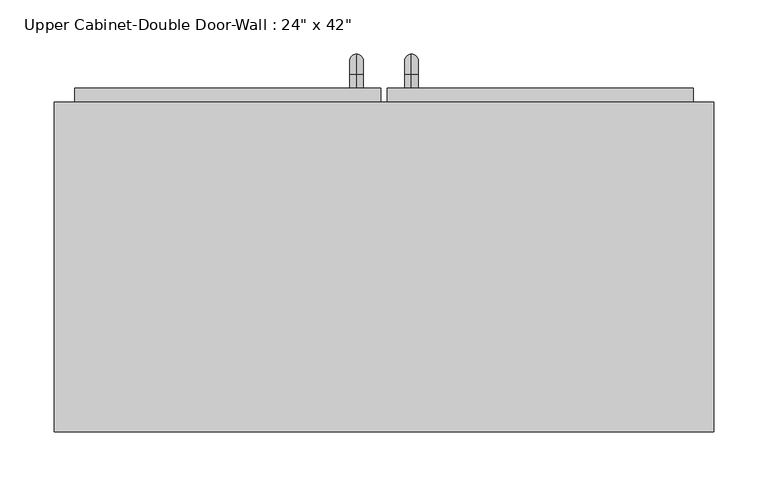
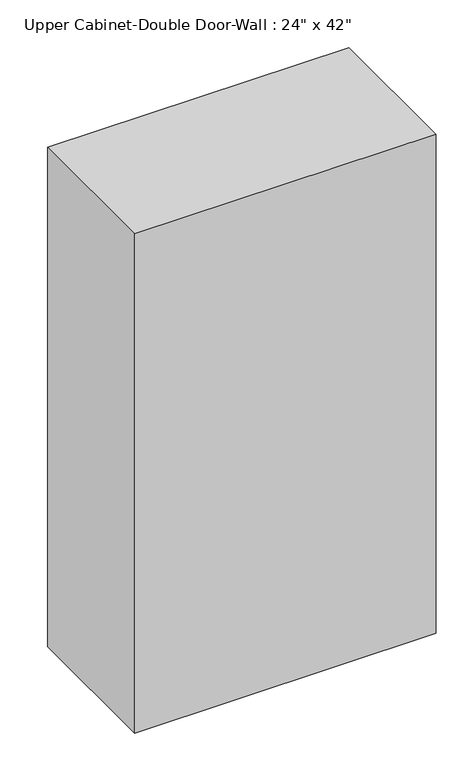
"""IFC4 building model written with IfcOpenShell, lengths in millimetres: furniture geometry."""

from ifc_helpers import new_model, si_unit, point, frame, origin, place, context, project, spatial, polyline, circle_curve, ellipse_curve, trimmed, outline, extrude, faceted_brep, source, transform, mapped, element, save
from ifc_brep_helpers import plane_surface, cylinder_surface, revolved_surface, advanced_brep


def furniture_7ad92d76(model_context):
    return source(origin(), model_context, "Body", "SolidModel", [
        faceted_brep([(-275.0288372, 61.9125, 2438.4), (-275.0288372, 61.9125, 1371.6), (334.5711628, 61.9125, 1371.6), (334.5711628, 61.9125, 2438.4), (-275.0288372, 366.7125, 2438.4), (334.5711628, 366.7125, 2438.4), (334.5711628, 366.7125, 1371.6), (-275.0288372, 366.7125, 1371.6), (-255.9788372, 366.7125, 2419.35), (-255.9788372, 366.7125, 1390.65), (315.5211628, 366.7125, 1390.65), (315.5211628, 366.7125, 2419.35), (315.5211628, 80.9625, 2419.35), (-255.9788372, 80.9625, 2419.35), (315.5211628, 80.9625, 1390.65), (-255.9788372, 80.9625, 1390.65)], [[[0, 1, 2, 3]], [[4, 5, 6, 7], [8, 9, 10, 11]], [[1, 0, 4, 7]], [[2, 1, 7, 6]], [[3, 2, 6, 5]], [[0, 3, 5, 4]], [[8, 11, 12, 13]], [[11, 10, 14, 12]], [[10, 9, 15, 14]], [[9, 8, 13, 15]], [[13, 12, 14, 15]]]),
        advanced_brep(
        [(55.1711628, 379.4125, 1517.65), (55.1711628, 379.4125, 1530.35), (55.1711628, 392.1125, 1517.65), (55.1711628, 392.1125, 1530.35), (55.1711628, 411.1625, 1511.3), (55.1711628, 398.4625, 1511.3), (55.1711628, 398.4625, 1435.1), (55.1711628, 411.1625, 1435.1), (55.1711628, 392.1125, 1416.05), (55.1711628, 392.1125, 1428.75), (55.1711628, 379.4125, 1428.75), (55.1711628, 379.4125, 1416.05)],
        [
            (0, 1, circle_curve(frame((55.1711628, 379.4125, 1524.0), z_axis=(0.0, -1.0, 0.0), x_axis=(0.0, 0.0, -1.0)), 6.35)),
            (1, 0, circle_curve(frame((55.1711628, 379.4125, 1524.0), z_axis=(0.0, -1.0, 0.0), x_axis=(0.0, 0.0, -1.0)), 6.35)),
            (0, 2),
            (2, 3, circle_curve(frame((55.1711628, 392.1125, 1524.0), z_axis=(0.0, -1.0, 0.0), x_axis=(0.0, 0.0, -1.0)), 6.35)),
            (3, 1),
            (3, 2, circle_curve(frame((55.1711628, 392.1125, 1524.0), z_axis=(0.0, -1.0, 0.0), x_axis=(0.0, 0.0, -1.0)), 6.35)),
            (4, 3, circle_curve(frame((55.1711628, 392.1125, 1511.3), z_axis=(1.0, 0.0, 0.0), x_axis=(0.0, 0.0, 1.0)), 19.05)),
            (2, 5, circle_curve(frame((55.1711628, 392.1125, 1511.3), z_axis=(-1.0, 0.0, 0.0), x_axis=(0.0, 0.0, 1.0)), 6.35)),
            (5, 4, circle_curve(frame((55.1711628, 404.8125, 1511.3), z_axis=(0.0, 0.0, 1.0), x_axis=(0.0, -1.0, 0.0)), 6.35)),
            (4, 5, circle_curve(frame((55.1711628, 404.8125, 1511.3), z_axis=(0.0, 0.0, 1.0), x_axis=(0.0, -1.0, 0.0)), 6.35)),
            (5, 6),
            (6, 7, circle_curve(frame((55.1711628, 404.8125, 1435.1), z_axis=(0.0, 0.0, 1.0), x_axis=(0.0, -1.0, 0.0)), 6.35)),
            (7, 4),
            (7, 6, circle_curve(frame((55.1711628, 404.8125, 1435.1), z_axis=(0.0, 0.0, 1.0), x_axis=(0.0, -1.0, 0.0)), 6.35)),
            (8, 7, circle_curve(frame((55.1711628, 392.1125, 1435.1), z_axis=(1.0, 0.0, 0.0), x_axis=(0.0, 1.0, 0.0)), 19.05)),
            (6, 9, circle_curve(frame((55.1711628, 392.1125, 1435.1), z_axis=(-1.0, 0.0, 0.0), x_axis=(0.0, 1.0, 0.0)), 6.35)),
            (9, 8, circle_curve(frame((55.1711628, 392.1125, 1422.4), z_axis=(0.0, 1.0, 0.0), x_axis=(0.0, 0.0, 1.0)), 6.35)),
            (8, 9, circle_curve(frame((55.1711628, 392.1125, 1422.4), z_axis=(0.0, 1.0, 0.0), x_axis=(0.0, 0.0, 1.0)), 6.35)),
            (10, 11, circle_curve(frame((55.1711628, 379.4125, 1422.4), z_axis=(0.0, -1.0, 0.0), x_axis=(0.0, 0.0, 1.0)), 6.35)),
            (11, 10, circle_curve(frame((55.1711628, 379.4125, 1422.4), z_axis=(0.0, -1.0, 0.0), x_axis=(0.0, 0.0, 1.0)), 6.35)),
            (9, 10),
            (11, 8),
        ],
        [
            plane_surface(frame((48.8211628, 379.4125, 1524.0), z_axis=(0.0, -1.0, 0.0), x_axis=(0.0, 0.0, 1.0))),
            cylinder_surface(frame((55.1711628, 379.4125, 1524.0), z_axis=(0.0, -1.0, 0.0), x_axis=(0.0, 0.0, -1.0)), 6.35),
            revolved_surface(trimmed(ellipse_curve(frame((55.1711628, 392.1125, 1524.0), z_axis=(0.0, -1.0, 0.0), x_axis=(0.0, 0.0, -1.0)), 6.35, 6.35), [point((55.1711628, 392.1125, 1517.65))], [point((55.1711628, 392.1125, 1530.35))], True, "CARTESIAN"), (55.1711628, 392.1125, 1511.3), (-1.0, 0.0, 0.0)),
            revolved_surface(trimmed(ellipse_curve(frame((55.1711628, 392.1125, 1524.0), z_axis=(0.0, -1.0, 0.0), x_axis=(0.0, 0.0, -1.0)), 6.35, 6.35), [point((55.1711628, 392.1125, 1530.35))], [point((55.1711628, 392.1125, 1517.65))], True, "CARTESIAN"), (55.1711628, 392.1125, 1511.3), (-1.0, 0.0, 0.0)),
            cylinder_surface(frame((55.1711628, 404.8125, 1511.3), z_axis=(0.0, 0.0, 1.0), x_axis=(0.0, -1.0, 0.0)), 6.35),
            revolved_surface(trimmed(ellipse_curve(frame((55.1711628, 404.8125, 1435.1), z_axis=(0.0, 0.0, 1.0), x_axis=(0.0, -1.0, 0.0)), 6.35, 6.35), [point((55.1711628, 398.4625, 1435.1))], [point((55.1711628, 411.1625, 1435.1))], True, "CARTESIAN"), (55.1711628, 392.1125, 1435.1), (-1.0, 0.0, 0.0)),
            revolved_surface(trimmed(ellipse_curve(frame((55.1711628, 404.8125, 1435.1), z_axis=(0.0, 0.0, 1.0), x_axis=(0.0, -1.0, 0.0)), 6.35, 6.35), [point((55.1711628, 411.1625, 1435.1))], [point((55.1711628, 398.4625, 1435.1))], True, "CARTESIAN"), (55.1711628, 392.1125, 1435.1), (-1.0, 0.0, 0.0)),
            plane_surface(frame((48.8211628, 379.4125, 1422.4), z_axis=(0.0, -1.0, 0.0), x_axis=(0.0, 0.0, -1.0))),
            cylinder_surface(frame((55.1711628, 392.1125, 1422.4), z_axis=(0.0, 1.0, 0.0), x_axis=(0.0, 0.0, 1.0)), 6.35),
        ],
        [
            (0, [[1, 2]]),
            (1, [[-1, 3, 4, 5]]),
            (1, [[-2, -5, 6, -3]]),
            (2, [[7, -4, 8, 9]]),
            (3, [[-8, -6, -7, 10]]),
            (4, [[-9, 11, 12, 13]]),
            (4, [[-10, -13, 14, -11]]),
            (5, [[15, -12, 16, 17]]),
            (6, [[-16, -14, -15, 18]]),
            (7, [[19, 20]]),
            (8, [[-17, 21, -20, 22]]),
            (8, [[-18, -22, -19, -21]]),
        ],
    ),
        advanced_brep(
        [(4.3711628, 379.4125, 1517.65), (4.3711628, 379.4125, 1530.35), (4.3711628, 392.1125, 1517.65), (4.3711628, 392.1125, 1530.35), (4.3711628, 411.1625, 1511.3), (4.3711628, 398.4625, 1511.3), (4.3711628, 398.4625, 1435.1), (4.3711628, 411.1625, 1435.1), (4.3711628, 392.1125, 1416.05), (4.3711628, 392.1125, 1428.75), (4.3711628, 379.4125, 1428.75), (4.3711628, 379.4125, 1416.05)],
        [
            (0, 1, circle_curve(frame((4.3711628, 379.4125, 1524.0), z_axis=(0.0, -1.0, 0.0), x_axis=(0.0, 0.0, 1.0)), 6.35)),
            (1, 0, circle_curve(frame((4.3711628, 379.4125, 1524.0), z_axis=(0.0, -1.0, 0.0), x_axis=(0.0, 0.0, 1.0)), 6.35)),
            (0, 2),
            (2, 3, circle_curve(frame((4.3711628, 392.1125, 1524.0), z_axis=(0.0, -1.0, 0.0), x_axis=(0.0, 0.0, 1.0)), 6.35)),
            (3, 1),
            (3, 2, circle_curve(frame((4.3711628, 392.1125, 1524.0), z_axis=(0.0, -1.0, 0.0), x_axis=(0.0, 0.0, 1.0)), 6.35)),
            (4, 3, circle_curve(frame((4.3711628, 392.1125, 1511.3), z_axis=(1.0, 0.0, 0.0), x_axis=(0.0, 0.0, 1.0)), 19.05)),
            (2, 5, circle_curve(frame((4.3711628, 392.1125, 1511.3), z_axis=(-1.0, 0.0, 0.0), x_axis=(0.0, 0.0, 1.0)), 6.35)),
            (5, 4, circle_curve(frame((4.3711628, 404.8125, 1511.3), z_axis=(0.0, 0.0, 1.0), x_axis=(0.0, 1.0, 0.0)), 6.35)),
            (4, 5, circle_curve(frame((4.3711628, 404.8125, 1511.3), z_axis=(0.0, 0.0, 1.0), x_axis=(0.0, 1.0, 0.0)), 6.35)),
            (5, 6),
            (6, 7, circle_curve(frame((4.3711628, 404.8125, 1435.1), z_axis=(0.0, 0.0, 1.0), x_axis=(0.0, 1.0, 0.0)), 6.35)),
            (7, 4),
            (7, 6, circle_curve(frame((4.3711628, 404.8125, 1435.1), z_axis=(0.0, 0.0, 1.0), x_axis=(0.0, 1.0, 0.0)), 6.35)),
            (8, 7, circle_curve(frame((4.3711628, 392.1125, 1435.1), z_axis=(1.0, 0.0, 0.0), x_axis=(0.0, 1.0, 0.0)), 19.05)),
            (6, 9, circle_curve(frame((4.3711628, 392.1125, 1435.1), z_axis=(-1.0, 0.0, 0.0), x_axis=(0.0, 1.0, 0.0)), 6.35)),
            (9, 8, circle_curve(frame((4.3711628, 392.1125, 1422.4), z_axis=(0.0, 1.0, 0.0), x_axis=(0.0, 0.0, -1.0)), 6.35)),
            (8, 9, circle_curve(frame((4.3711628, 392.1125, 1422.4), z_axis=(0.0, 1.0, 0.0), x_axis=(0.0, 0.0, -1.0)), 6.35)),
            (10, 11, circle_curve(frame((4.3711628, 379.4125, 1422.4), z_axis=(0.0, -1.0, 0.0), x_axis=(0.0, 0.0, -1.0)), 6.35)),
            (11, 10, circle_curve(frame((4.3711628, 379.4125, 1422.4), z_axis=(0.0, -1.0, 0.0), x_axis=(0.0, 0.0, -1.0)), 6.35)),
            (9, 10),
            (11, 8),
        ],
        [
            plane_surface(frame((-1.9788372, 379.4125, 1524.0), z_axis=(0.0, -1.0, 0.0), x_axis=(0.0, 0.0, 1.0))),
            cylinder_surface(frame((4.3711628, 379.4125, 1524.0), z_axis=(0.0, -1.0, 0.0), x_axis=(0.0, 0.0, 1.0)), 6.35),
            revolved_surface(trimmed(ellipse_curve(frame((4.3711628, 392.1125, 1524.0), z_axis=(0.0, -1.0, 0.0), x_axis=(0.0, 0.0, 1.0)), 6.35, 6.35), [point((4.3711628, 392.1125, 1517.65))], [point((4.3711628, 392.1125, 1530.35))], True, "CARTESIAN"), (4.3711628, 392.1125, 1511.3), (-1.0, 0.0, 0.0)),
            revolved_surface(trimmed(ellipse_curve(frame((4.3711628, 392.1125, 1524.0), z_axis=(0.0, -1.0, 0.0), x_axis=(0.0, 0.0, 1.0)), 6.35, 6.35), [point((4.3711628, 392.1125, 1530.35))], [point((4.3711628, 392.1125, 1517.65))], True, "CARTESIAN"), (4.3711628, 392.1125, 1511.3), (-1.0, 0.0, 0.0)),
            cylinder_surface(frame((4.3711628, 404.8125, 1511.3), z_axis=(0.0, 0.0, 1.0), x_axis=(0.0, 1.0, 0.0)), 6.35),
            revolved_surface(trimmed(ellipse_curve(frame((4.3711628, 404.8125, 1435.1), z_axis=(0.0, 0.0, 1.0), x_axis=(0.0, 1.0, 0.0)), 6.35, 6.35), [point((4.3711628, 398.4625, 1435.1))], [point((4.3711628, 411.1625, 1435.1))], True, "CARTESIAN"), (4.3711628, 392.1125, 1435.1), (-1.0, 0.0, 0.0)),
            revolved_surface(trimmed(ellipse_curve(frame((4.3711628, 404.8125, 1435.1), z_axis=(0.0, 0.0, 1.0), x_axis=(0.0, 1.0, 0.0)), 6.35, 6.35), [point((4.3711628, 411.1625, 1435.1))], [point((4.3711628, 398.4625, 1435.1))], True, "CARTESIAN"), (4.3711628, 392.1125, 1435.1), (-1.0, 0.0, 0.0)),
            plane_surface(frame((-1.9788372, 379.4125, 1422.4), z_axis=(0.0, -1.0, 0.0), x_axis=(0.0, 0.0, -1.0))),
            cylinder_surface(frame((4.3711628, 392.1125, 1422.4), z_axis=(0.0, 1.0, 0.0), x_axis=(0.0, 0.0, -1.0)), 6.35),
        ],
        [
            (0, [[1, 2]]),
            (1, [[-1, 3, 4, 5]]),
            (1, [[-2, -5, 6, -3]]),
            (2, [[7, -4, 8, 9]]),
            (3, [[-8, -6, -7, 10]]),
            (4, [[-9, 11, 12, 13]]),
            (4, [[-10, -13, 14, -11]]),
            (5, [[15, -12, 16, 17]]),
            (6, [[-16, -14, -15, 18]]),
            (7, [[19, 20]]),
            (8, [[-17, 21, -20, 22]]),
            (8, [[-18, -22, -19, -21]]),
        ],
    ),
        extrude(outline(polyline([(32.9461628, 379.4125), (315.5211628, 379.4125), (315.5211628, 347.6625), (32.9461628, 347.6625), (32.9461628, 379.4125)])), frame((0.0, 0.0, 1390.65), z_axis=(0.0, 0.0, 1.0), x_axis=(1.0, 0.0, 0.0)), (0.0, 0.0, 1.0), 1028.7),
        extrude(outline(polyline([(-255.9788372, 379.4125), (26.5961628, 379.4125), (26.5961628, 347.6625), (-255.9788372, 347.6625), (-255.9788372, 379.4125)])), frame((0.0, 0.0, 1390.65), z_axis=(0.0, 0.0, 1.0), x_axis=(1.0, 0.0, 0.0)), (0.0, 0.0, 1.0), 1028.7),
    ])


if __name__ == "__main__":
    model = new_model("IFC4")
    model_context = context("Model", 3, world=origin())
    ifc_project = project(units=[si_unit("LENGTHUNIT", "METRE", prefix="MILLI")], contexts=[model_context])
    site = spatial("IfcSite", under=ifc_project)
    building = spatial("IfcBuilding", under=site)
    placement = place(None, origin())
    furniture_shape = furniture_7ad92d76(model_context)
    element("IfcFurniture", 1, ObjectType="Upper Cabinet-Double Door-Wall : 24\" x 42\"", at=placement, inside=building, context=model_context, shape_type="MappedRepresentation", body=[
        mapped(furniture_shape, transform((0.0, 0.0, 0.0), x_axis=(1.0, 0.0, 0.0), y_axis=(0.0, 1.0, 0.0), z_axis=(0.0, 0.0, 1.0))),
    ])
    save(model, "model.ifc")

# Revit data of these elements
# Type "Upper Cabinet-Double Door-Wall : 24\" x 42\""
#   COBie.Type.CreatedBy = "doug.wood@us.ibm.com"
#   COBie.Type.CreatedOn = "2016-04-14T02:07:23"
#   COBie.Type.Name = "Casework_Upper Cabinet-Double Door-Wall_24\" x 42\""
#   COBie.Type.Category = "23-40 35 17 47 11 : Kitchen Casework"
#   COBie.Type.Description = "Upper Cabinet-Double Door-Wall_24\" x 42\""
#   COBie.Type.Manufacturer = ""
#   COBie.Type.ModelNumber = ""
#   Assembly Code = "C1030410"
#   COBie.Type.ReplacementCost = 0
#   Depth = 1' - 0"
#   Height = 3' - 6"
#   Top Of Cabinet = 8' - 0"
#   Width = 2' - 0"
#   COBie.Type = no
#   Cabinet Material = none
#   Door/Drawer Material = none
#   Handle Material = Cabinets - Handles
# Element 1 (IfcFurniture, "Upper Cabinet-Double Door-Wall : 24\" x 42\"")
#   Materials on its faces: "Cabinets - Handles", "Cabinets"
# Materials
#   "Cabinets - Handles": class "Metal", colour RGB 57 57 57, transparency 0
#   "Cabinets": class "Miscellaneous", colour RGB 249 249 249, transparency 0
